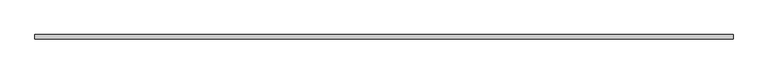
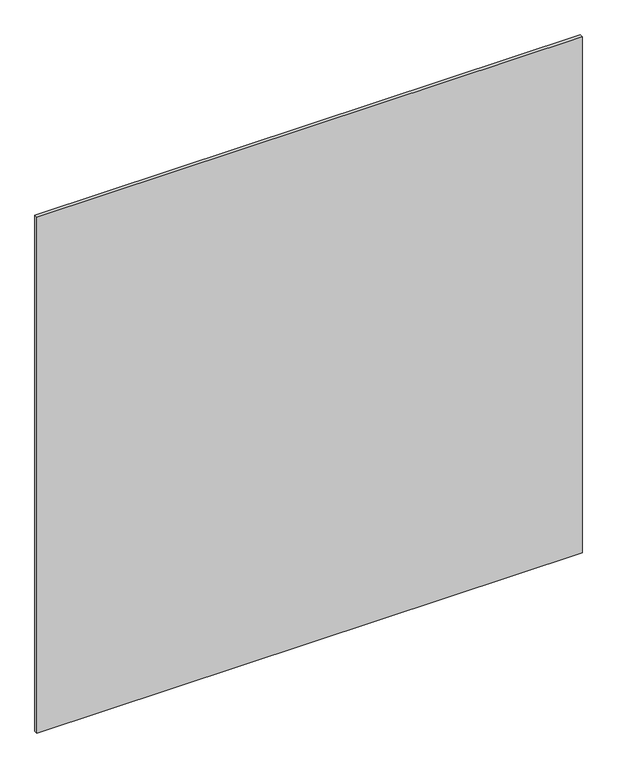
"""IFC4 building model written with IfcOpenShell, lengths in millimetres: proxy geometry, Panel:Panel:300402:Panel:300402 : Panel:Panel:300402:300124:Panel:300402:Panel:300402 : Panel:Panel:300402:300124 : Panel:Panel:300402:Panel:300402 : Panel:Panel:300402:300124:4 : Panel:Panel:300402:Panel:300402 : Panel:Panel:300402:300124:Panel:300402:Panel:300402 : Panel:Panel:300402:300124 : Panel:Panel:300402:Panel:300402 : Panel:Panel:300402:300124:300083."""

from ifc_helpers import new_model, si_unit, frame, origin, place, context, project, spatial, polyline, outline, extrude, source, transform, mapped, element, save


def generic_models_96526297(model_context):
    return source(origin(), model_context, "Body", "SweptSolid", [
        extrude(outline(polyline([(570452.6367239, -579076.8913841), (571671.8367239, -579076.8913841), (571671.8367239, -579084.8288841), (570452.6367239, -579084.8288841), (570452.6367239, -579076.8913841)])), frame((0.0, 0.0, 4914.9), z_axis=(0.0, 0.0, 1.0), x_axis=(1.0, 0.0, 0.0)), (0.0, 0.0, 1.0), 1219.2),
    ])


if __name__ == "__main__":
    model = new_model("IFC4")
    model_context = context("Model", 3, world=origin())
    ifc_project = project(units=[si_unit("LENGTHUNIT", "METRE", prefix="MILLI")], contexts=[model_context])
    site = spatial("IfcSite", under=ifc_project)
    building = spatial("IfcBuilding", under=site)
    placement = place(None, origin())
    generic_models_shape = generic_models_96526297(model_context)
    element("IfcBuildingElementProxy", 1, Name="Panel:Panel:300402:Panel:300402 : Panel:Panel:300402:300124:Panel:300402:Panel:300402 : Panel:Panel:300402:300124 : Panel:Panel:300402:Panel:300402 : Panel:Panel:300402:300124:4 : Panel:Panel:300402:Panel:300402 : Panel:Panel:300402:300124:Panel:300402:Panel:300402 : Panel:Panel:300402:300124 : Panel:Panel:300402:Panel:300402 : Panel:Panel:300402:300124:300083", ObjectType="Panel:Panel:300402:Panel:300402 : Panel:Panel:300402:300124:Panel:300402:Panel:300402 : Panel:Panel:300402:300124 : Panel:Panel:300402:Panel:300402 : Panel:Panel:300402:300124:4 : Panel:Panel:300402:Panel:300402 : Panel:Panel:300402:300124:Panel:300402:Panel:300402 : Panel:Panel:300402:300124 : Panel:Panel:300402:Panel:300402 : Panel:Panel:300402:300124:300083", at=placement, inside=building, context=model_context, shape_type="MappedRepresentation", body=[
        mapped(generic_models_shape, transform((0.0, 0.0, 0.0), x_axis=(1.0, 0.0, 0.0), y_axis=(0.0, 1.0, 0.0), z_axis=(0.0, 0.0, 1.0))),
    ])
    save(model, "model.ifc")

# Revit data of these elements
# Type "Panel:Panel:300402:Panel:300402 : Panel:Panel:300402:300124:Panel:300402:Panel:300402 : Panel:Panel:300402:300124 : Panel:Panel:300402:Panel:300402 : Panel:Panel:300402:300124:4 : Panel:Panel:300402:Panel:300402 : Panel:Panel:300402:300124:Panel:300402:Panel:300402 : Panel:Panel:300402:300124 : Panel:Panel:300402:Panel:300402 : Panel:Panel:300402:300124:300083"
#   NameOverride = "Panel:Panel:300402:Panel:300402 : Panel:Panel:300402:300124:Panel:300402:Panel:300402 : Panel:Panel:300402:300124 : Panel:Panel:300402:Panel:300402 : Panel:Panel:300402:300124:300083"
#   ObjectTypeOverride = "Panel:300402:Panel:300402 : Panel:Panel:300402:300124 : Panel:Panel:300402:Panel:300402 : Panel:Panel:300402:300124"
#   Reference = "Panel"
#   Tag = "300083"
# Element 1 (IfcBuildingElementProxy, "Panel:Panel:300402:Panel:300402 : Panel:Panel:300402:300124:Panel:300402:Panel:300402 : Panel:Panel:300402:300124 : Panel:Panel:300402:Panel:300402 : Panel:Panel:300402:300124:4 : Panel:Panel:300402:Panel:300402 : Panel:Panel:300402:300124:Panel:300402:Panel:300402 : Panel:Panel:300402:300124 : Panel:Panel:300402:Panel:300402 : Panel:Panel:300402:300124:300083")
#   Materials on its faces: "5/16\" PHENOLIC RESIN PANELS (CLASS A FLAME SPREAD) - EXPOSED FASTENERS"
# Materials
#   "5/16\" PHENOLIC RESIN PANELS (CLASS A FLAME SPREAD) - EXPOSED FASTENERS": class "Unassigned", colour RGB 64 64 64, transparency 0, Keynote = "M07420000.01", Cost = 0
